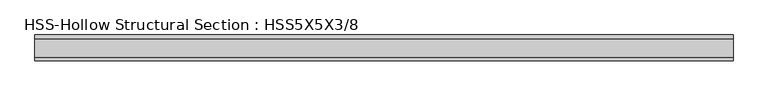
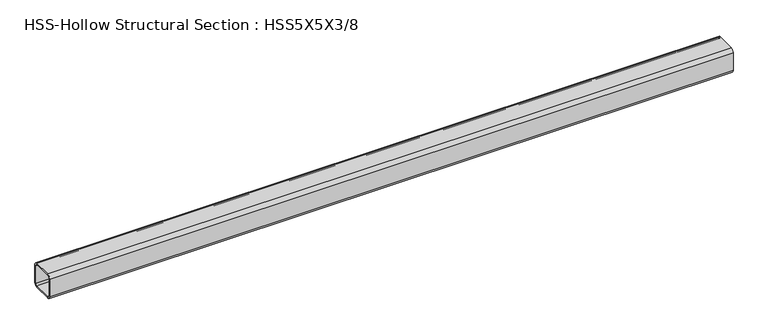
"""IFC4 building model written with IfcOpenShell, lengths in millimetres: member geometry, HSS-Hollow Structural Section : HSS5X5X3/8."""

from ifc_helpers import new_model, si_unit, point, frame, frame_2d, origin, place, context, project, spatial, polyline, circle_curve, trimmed, segment, composite_curve, outline, extrude, source, transform, mapped, element, save


def hss_hollow_structural_section_hss5x5x3_8_8075c1df(model_context):
    return source(origin(), model_context, "Body", "SweptSolid", [
        extrude(outline(composite_curve([segment(polyline([(63.5, 45.7708), (63.5, -45.7708)]), True, "CONTINUOUS"), segment(trimmed(circle_curve(frame_2d((45.7708, -45.7708)), 17.7292), [point((63.5, -45.7708))], [point((45.7708, -63.5))], False, "CARTESIAN"), True, "CONTINUOUS"), segment(polyline([(45.7708, -63.5), (-45.7708, -63.5)]), True, "CONTINUOUS"), segment(trimmed(circle_curve(frame_2d((-45.7708, -45.7708)), 17.7292), [point((-45.7708, -63.5))], [point((-63.5, -45.7708))], False, "CARTESIAN"), True, "CONTINUOUS"), segment(polyline([(-63.5, -45.7708), (-63.5, 45.7708)]), True, "CONTINUOUS"), segment(trimmed(circle_curve(frame_2d((-45.7708, 45.7708)), 17.7292), [point((-63.5, 45.7708))], [point((-45.7708, 63.5))], False, "CARTESIAN"), True, "CONTINUOUS"), segment(polyline([(-45.7708, 63.5), (45.7708, 63.5)]), True, "CONTINUOUS"), segment(trimmed(circle_curve(frame_2d((45.7708, 45.7708)), 17.7292), [point((45.7708, 63.5))], [point((63.5, 45.7708))], False, "CARTESIAN"), True, "CONTINUOUS")], self_intersect=False), holes=[composite_curve([segment(trimmed(circle_curve(frame_2d((-45.7708, 45.7708)), 8.8646), [point((-45.7708, 54.6354))], [point((-54.6354, 45.7708))], True, "CARTESIAN"), True, "CONTINUOUS"), segment(polyline([(-54.6354, 45.7708), (-54.6354, -45.7708)]), True, "CONTINUOUS"), segment(trimmed(circle_curve(frame_2d((-45.7708, -45.7708)), 8.8646), [point((-54.6354, -45.7708))], [point((-45.7708, -54.6354))], True, "CARTESIAN"), True, "CONTINUOUS"), segment(polyline([(-45.7708, -54.6354), (45.7708, -54.6354)]), True, "CONTINUOUS"), segment(trimmed(circle_curve(frame_2d((45.7708, -45.7708)), 8.8646), [point((45.7708, -54.6354))], [point((54.6354, -45.7708))], True, "CARTESIAN"), True, "CONTINUOUS"), segment(polyline([(54.6354, -45.7708), (54.6354, 45.7708)]), True, "CONTINUOUS"), segment(trimmed(circle_curve(frame_2d((45.7708, 45.7708)), 8.8646), [point((54.6354, 45.7708))], [point((45.7708, 54.6354))], True, "CARTESIAN"), True, "CONTINUOUS"), segment(polyline([(45.7708, 54.6354), (-45.7708, 54.6354)]), True, "CONTINUOUS")], self_intersect=False)]), frame((-1700.4138997, 0.0, 0.0), z_axis=(1.0, 0.0, 0.0), x_axis=(0.0, 1.0, 0.0)), (0.0, 0.0, 1.0), 3400.8277993),
    ])


if __name__ == "__main__":
    model = new_model("IFC4")
    model_context = context("Model", 3, world=origin())
    ifc_project = project(units=[si_unit("LENGTHUNIT", "METRE", prefix="MILLI")], contexts=[model_context])
    site = spatial("IfcSite", under=ifc_project)
    building = spatial("IfcBuilding", under=site)
    placement = place(None, origin())
    hss_hollow_structural_section_hss5x5x3_8_shape = hss_hollow_structural_section_hss5x5x3_8_8075c1df(model_context)
    element("IfcMember", 1, ObjectType="HSS-Hollow Structural Section : HSS5X5X3/8", at=placement, inside=building, context=model_context, shape_type="MappedRepresentation", body=[
        mapped(hss_hollow_structural_section_hss5x5x3_8_shape, transform((0.0, 0.0, 0.0), x_axis=(1.0, 0.0, 0.0), y_axis=(0.0, 1.0, 0.0), z_axis=(0.0, 0.0, 1.0))),
    ])
    save(model, "model.ifc")

# Revit data of these elements
# Type "HSS-Hollow Structural Section : HSS5X5X3/8"
#   Assembly Code = "B10"
#   Shape = "Square"
#   W = 22.3
#   Ht = 0' - 5"
#   Length [instance default] = 5' - 0"
#   b = 0' - 5"
#   kr = 0' - 0.698"
#   t = 0' - 0.349"
#   A = 0.0429167 SF
#   Structural Material [instance default] = Steel ASTM A500, Grade B, Rectangular and Square
# Element 1 (IfcMember, "HSS-Hollow Structural Section : HSS5X5X3/8")
#   Materials on its faces: "Steel ASTM A500, Grade B, Rectangular and Square"
# Materials
#   "Steel ASTM A500, Grade B, Rectangular and Square": class "Metal", colour RGB 199 199 199, transparency 0, Description = "Carbon steel", Cost = 0
